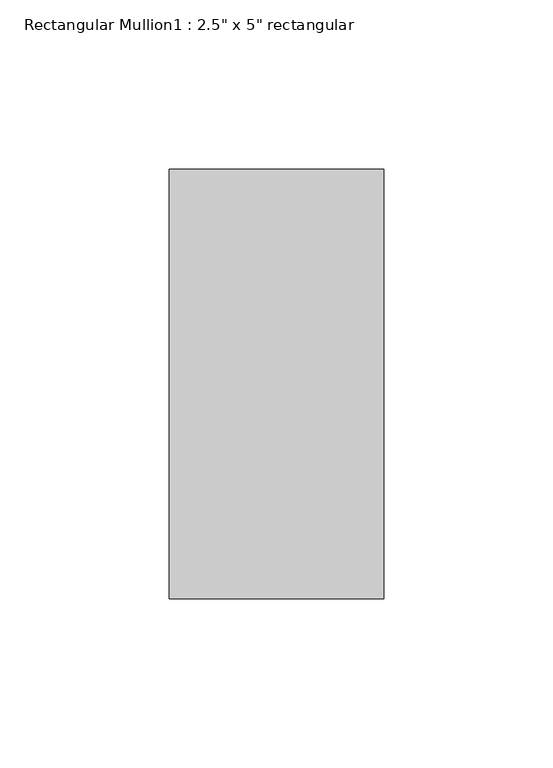
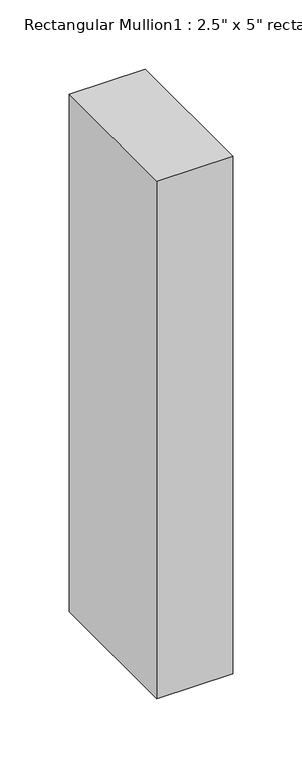
"""IFC4 building model written with IfcOpenShell, lengths in millimetres: member geometry."""

from ifc_helpers import new_model, si_unit, frame, origin, place, context, project, spatial, polyline, outline, extrude, source, transform, mapped, element, save


def member_ffd4c858(model_context):
    return source(origin(), model_context, "Body", "SweptSolid", [
        extrude(outline(polyline([(31.75, 63.5), (31.75, -63.5), (-31.75, -63.5), (-31.75, 63.5), (31.75, 63.5)])), frame((0.0, 0.0, -457.2), z_axis=(0.0, 0.0, 1.0), x_axis=(1.0, 0.0, 0.0)), (0.0, 0.0, 1.0), 457.2),
    ])


if __name__ == "__main__":
    model = new_model("IFC4")
    model_context = context("Model", 3, world=origin())
    ifc_project = project(units=[si_unit("LENGTHUNIT", "METRE", prefix="MILLI")], contexts=[model_context])
    site = spatial("IfcSite", under=ifc_project)
    building = spatial("IfcBuilding", under=site)
    placement = place(None, origin())
    member_shape = member_ffd4c858(model_context)
    element("IfcMember", 1, ObjectType="Rectangular Mullion1 : 2.5\" x 5\" rectangular", at=placement, inside=building, context=model_context, shape_type="MappedRepresentation", body=[
        mapped(member_shape, transform((0.0, 0.0, 0.0), x_axis=(1.0, 0.0, 0.0), y_axis=(0.0, 1.0, 0.0), z_axis=(0.0, 0.0, 1.0))),
    ])
    save(model, "model.ifc")

# Revit data of these elements
# Type "Rectangular Mullion1 : 2.5\" x 5\" rectangular"
#   built-in parameter 1007304 = 0.416667 (stored number, unit not read)
#   built-in parameter 1007301 = 0.104167 (stored number, unit not read)
#   built-in parameter 1007300 = 0.104167 (stored number, unit not read)
# Element 1 (IfcMember, "Rectangular Mullion1 : 2.5\" x 5\" rectangular")
#   Materials on its faces: "support-frame"
# Materials
#   "support-frame": class "Unassigned", colour RGB 233 233 233, transparency 0, Cost = 0
